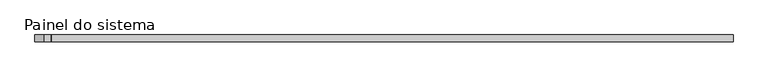
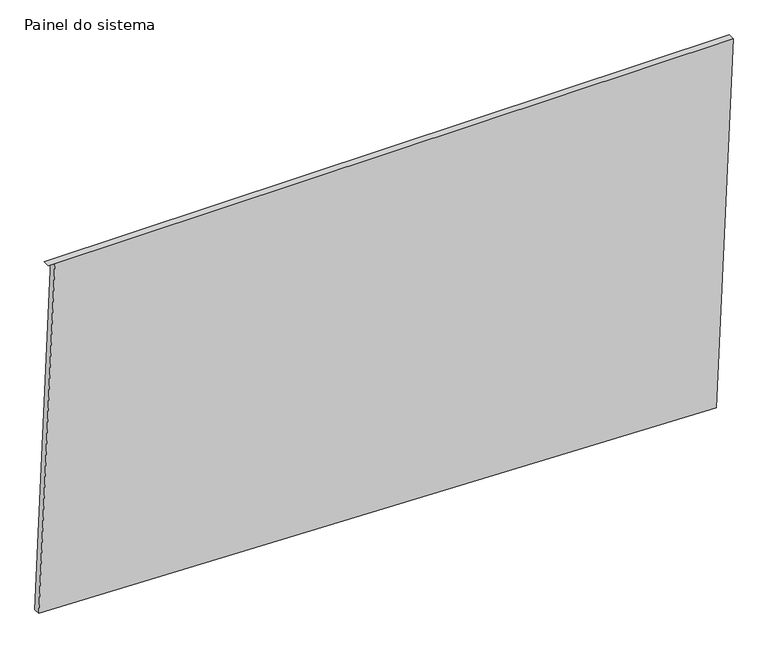
"""IFC4 building model written with IfcOpenShell, lengths in millimetres: plate geometry, Painel do sistema : Envidraçado."""

import ifcopenshell
import ifcopenshell.guid

model = None  # the IFC model being written
_history = None  # IfcOwnerHistory: only IFC2X3 demands one
_inside = {}  # id of a spatial element -> (the spatial element, [elements in it])
_under = {}  # id of a project, library or spatial element -> (it, [spatial elements below it])
_declared = {}  # id of a project -> (the project, [libraries it declares])
_typed = {}  # id of a type object -> (the type object, [elements of that type])
_made_of = {}  # id of a material, layer set ... -> (it, [elements and type objects made of it])


def new_model(schema):
    """Start an empty IFC model of exactly this schema.

    Asked for "IFC4X3", IfcOpenShell would pick the latest addendum, in which some entities
    have other attributes; the version numbers below select the first issue.
    IFC2X3 requires an IfcOwnerHistory on every rooted entity: one is made here for all.
    """
    global model, _history
    if schema == "IFC4X3":
        model = ifcopenshell.file(schema_version=(4, 3, 0, 0))
    else:
        model = ifcopenshell.file(schema=schema)
    _inside.clear()
    _under.clear()
    _declared.clear()
    _typed.clear()
    _made_of.clear()
    _history = None
    if model.schema == "IFC2X3":
        org = make("IfcOrganization", Name="unknown")
        user = make(
            "IfcPersonAndOrganization",
            ThePerson=make("IfcPerson", FamilyName="unknown"),
            TheOrganization=org,
        )
        app = make(
            "IfcApplication",
            ApplicationDeveloper=org,
            Version="unknown",
            ApplicationFullName="unknown",
            ApplicationIdentifier="unknown",
        )
        _history = make(
            "IfcOwnerHistory",
            OwningUser=user,
            OwningApplication=app,
            ChangeAction="ADDED",
            CreationDate=0,
        )
    return model


def make(cls, **values):
    """One entity of the class cls with the attributes given. An attribute that is None is left unset."""
    return model.create_entity(
        cls, **{name: value for name, value in values.items() if value is not None}
    )


def rooted(cls, **values):
    """An entity with a GlobalId (a new one), such as an element, a storey or a relation."""
    return make(cls, GlobalId=ifcopenshell.guid.new(), OwnerHistory=_history, **values)


def si_unit(unit_type, name, prefix=None):
    """IfcSIUnit, for example si_unit("LENGTHUNIT", "METRE", prefix="MILLI")."""
    return make("IfcSIUnit", UnitType=unit_type, Prefix=prefix, Name=name)


def assignment(units):
    """IfcUnitAssignment: the units of a project."""
    return None if units is None else make("IfcUnitAssignment", Units=units)


def point(xyz):
    """IfcCartesianPoint."""
    return None if xyz is None else make("IfcCartesianPoint", Coordinates=xyz)


def direction(xyz):
    """IfcDirection."""
    return None if xyz is None else make("IfcDirection", DirectionRatios=xyz)


def frame(location, z_axis=None, x_axis=None):
    """IfcAxis2Placement3D, a coordinate frame: its origin and axes. An axis left out is left unset."""
    return make(
        "IfcAxis2Placement3D",
        Location=point(location),
        Axis=direction(z_axis),
        RefDirection=direction(x_axis),
    )


def origin():
    """The frame at (0, 0, 0) with its axes left unset."""
    return frame((0.0, 0.0, 0.0))


def place(relative_to, where):
    """IfcLocalPlacement: puts the frame where relative to a parent placement (None: the world)."""
    return make(
        "IfcLocalPlacement", PlacementRelTo=relative_to, RelativePlacement=where
    )


def context(
    kind, dimensions, precision=None, world=None, true_north=None, identifier=None
):
    """IfcGeometricRepresentationContext, for example the 3D "Model" context."""
    return make(
        "IfcGeometricRepresentationContext",
        ContextIdentifier=identifier,
        ContextType=kind,
        CoordinateSpaceDimension=dimensions,
        Precision=precision,
        WorldCoordinateSystem=world,
        TrueNorth=true_north,
    )


def project(units=None, contexts=None):
    """IfcProject with its units and contexts."""
    return rooted(
        "IfcProject",
        Name="project",
        RepresentationContexts=contexts,
        UnitsInContext=assignment(units),
    )


def spatial(cls, under=None, at=None, **own):
    """A site, building, storey or space (cls), placed at a placement, below another one or the project."""
    s = rooted(cls, ObjectPlacement=at, **own)
    if under is not None:
        _under.setdefault(under.id(), (under, []))[1].append(s)
    return s


def polyline(points):
    """IfcPolyline through the points."""
    return make("IfcPolyline", Points=[point(p) for p in points])


def outline(outer, holes=None, kind="AREA"):
    """IfcArbitraryClosedProfileDef: a profile drawn as a closed curve; with holes, ...WithVoids."""
    if holes is None:
        return make("IfcArbitraryClosedProfileDef", ProfileType=kind, OuterCurve=outer)
    return make(
        "IfcArbitraryProfileDefWithVoids",
        ProfileType=kind,
        OuterCurve=outer,
        InnerCurves=holes,
    )


def extrude(swept, where, along, depth):
    """IfcExtrudedAreaSolid: the profile swept, set in the frame where, extruded along a direction by depth."""
    return make(
        "IfcExtrudedAreaSolid",
        SweptArea=swept,
        Position=where,
        ExtrudedDirection=direction(along),
        Depth=depth,
    )


def shape(context_of_items, identifier, shape_type, items):
    """IfcShapeRepresentation: the items that make up one representation, for example the "Body"."""
    return make(
        "IfcShapeRepresentation",
        ContextOfItems=context_of_items,
        RepresentationIdentifier=identifier,
        RepresentationType=shape_type,
        Items=items,
    )


def source(mapping_origin, context_of_items, identifier, shape_type, items):
    """IfcRepresentationMap: a shape defined once, which mapped items show again and again."""
    return make(
        "IfcRepresentationMap",
        MappingOrigin=mapping_origin,
        MappedRepresentation=shape(context_of_items, identifier, shape_type, items),
    )


def transform(
    local_origin,
    x_axis=None,
    y_axis=None,
    z_axis=None,
    scale=None,
    scale2=None,
    scale3=None,
    uniform=True,
):
    """IfcCartesianTransformationOperator3D, or its non-uniform kind. x_axis, y_axis, z_axis: its Axis1, 2, 3."""
    if uniform:
        return make(
            "IfcCartesianTransformationOperator3D",
            Axis1=direction(x_axis),
            Axis2=direction(y_axis),
            LocalOrigin=point(local_origin),
            Scale=scale,
            Axis3=direction(z_axis),
        )
    return make(
        "IfcCartesianTransformationOperator3DnonUniform",
        Axis1=direction(x_axis),
        Axis2=direction(y_axis),
        LocalOrigin=point(local_origin),
        Scale=scale,
        Axis3=direction(z_axis),
        Scale2=scale2,
        Scale3=scale3,
    )


def mapped(mapping_source, mapping_target):
    """IfcMappedItem: shows the shape of a source again, moved by a transform."""
    return make(
        "IfcMappedItem", MappingSource=mapping_source, MappingTarget=mapping_target
    )


def made_of(thing, what):
    """Note that an element or type object is made of a material, layer set ...; save() writes the relation."""
    if what is not None:
        _made_of.setdefault(what.id(), (what, []))[1].append(thing)
    return thing


def element(
    cls,
    number,
    at=None,
    inside=None,
    cuts=None,
    type_object=None,
    material=None,
    context=None,
    identifier="Body",
    shape_type=None,
    held_by="IfcProductDefinitionShape",
    body=None,
    shapes=None,
    **own,
):
    """One element of the class cls, such as IfcWall. Its Tag is "e" and its number.

    at: its placement. inside: the storey or other place that contains it. cuts: it is an
    opening in that element (IfcRelVoidsElement). A single representation is given by context,
    identifier, shape_type and body (its items); several are given by shapes. held_by: the class
    of the entity that holds the representations. save() writes the other relations.
    """
    e = rooted(cls, Tag="e%d" % number, ObjectPlacement=at, **own)
    if body is not None:
        shapes = [shape(context, identifier, shape_type, body)]
    if shapes is not None:
        e.Representation = make(held_by, Representations=shapes)
    if inside is not None:
        _inside.setdefault(inside.id(), (inside, []))[1].append(e)
    if cuts is not None:
        rooted(
            "IfcRelVoidsElement", RelatingBuildingElement=cuts, RelatedOpeningElement=e
        )
    if type_object is not None:
        _typed.setdefault(type_object.id(), (type_object, []))[1].append(e)
    return made_of(e, material)


def aggregate(whole, parts):
    """IfcRelAggregates: a whole, such as a stair, and the parts it consists of."""
    return rooted("IfcRelAggregates", RelatingObject=whole, RelatedObjects=parts)


def save(model, path):
    """Write the relations noted so far, then the file.

    IfcRelAggregates (storeys below a building ...), IfcRelContainedInSpatialStructure (elements
    in a storey), IfcRelDefinesByType, IfcRelAssociatesMaterial and IfcRelDeclares: one each for
    every whole, place, type object, material and project.
    """
    for whole, parts in _under.values():
        aggregate(whole, parts)
    for where, things in _inside.values():
        rooted(
            "IfcRelContainedInSpatialStructure",
            RelatedElements=things,
            RelatingStructure=where,
        )
    for kind, things in _typed.values():
        rooted("IfcRelDefinesByType", RelatedObjects=things, RelatingType=kind)
    for what, things in _made_of.values():
        rooted("IfcRelAssociatesMaterial", RelatedObjects=things, RelatingMaterial=what)
    for by, libraries in _declared.values():
        rooted("IfcRelDeclares", RelatingContext=by, RelatedDefinitions=libraries)
    model.write(path)


def painel_do_sistema_b5435940(model_context):
    return source(origin(), model_context, "Body", "SweptSolid", [
        extrude(outline(polyline([(72.8211161, -1292.3421783), (0.0, 1229.5208981), (1429.8579776, 1292.3421783), (1429.8579776, -1257.7444351), (1428.760653, -1232.7685291), (72.8211161, -1292.3421783)])), frame((0.0, 24.5, 0.0), z_axis=(0.0, 1.0, 0.0), x_axis=(0.0, 0.0, 1.0)), (0.0, 0.0, 1.0), 25.0),
    ])


if __name__ == "__main__":
    model = new_model("IFC4")
    model_context = context("Model", 3, world=origin())
    ifc_project = project(units=[si_unit("LENGTHUNIT", "METRE", prefix="MILLI")], contexts=[model_context])
    site = spatial("IfcSite", under=ifc_project)
    building = spatial("IfcBuilding", under=site)
    placement = place(None, origin())
    painel_do_sistema_shape = painel_do_sistema_b5435940(model_context)
    element("IfcPlate", 1, ObjectType="Painel do sistema : Envidraçado", at=placement, inside=building, context=model_context, shape_type="MappedRepresentation", body=[
        mapped(painel_do_sistema_shape, transform((0.0, 0.0, 0.0), x_axis=(1.0, 0.0, 0.0), y_axis=(0.0, 1.0, 0.0), z_axis=(0.0, 0.0, 1.0))),
    ])
    save(model, "model.ifc")

# Revit data of these elements
# Type "Painel do sistema : Envidraçado"
#   Construction Type Id = "GSP4R"
#   Analytic Construction = "Vidraça única Pilkington 1/8 pol"
#   Visual Light Transmittance = 0.9
#   Solar Heat Gain Coefficient = 0.86
#   Heat Transfer Coefficient (U) = 6.7069 W/(m²·K)
# Element 1 (IfcPlate, "Painel do sistema : Envidraçado")
#   Materials on its faces: "Vidro"
# Materials
#   "Vidro": class "Vidro", colour RGB 0 128 192, transparency 0.9, Description = "Vidro de sílica", Cost = 0
